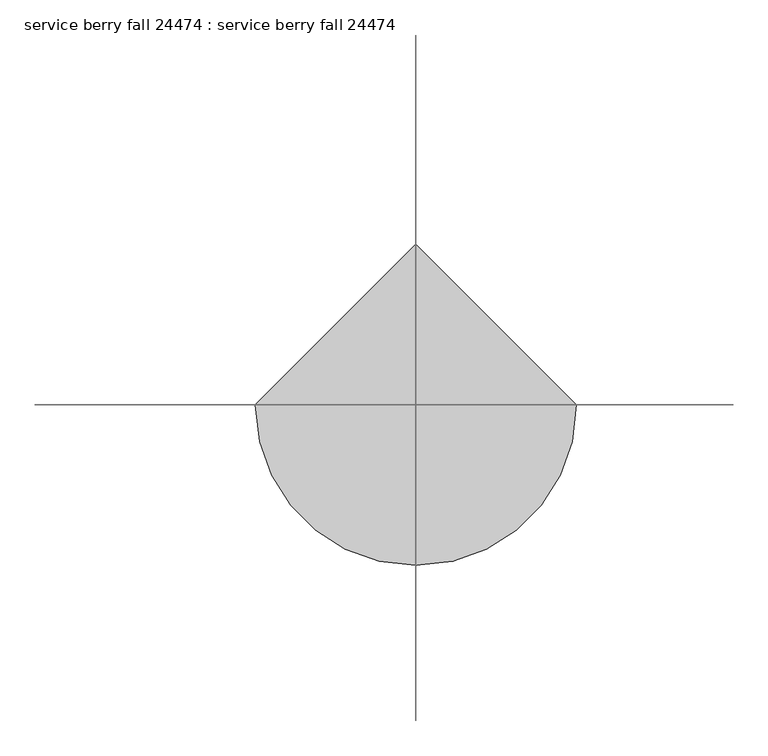
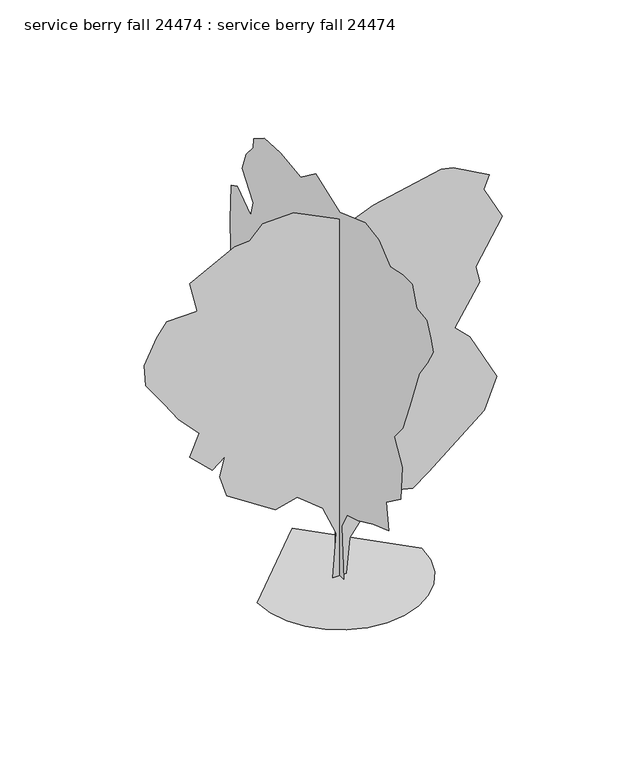
"""IFC4 building model written with IfcOpenShell, lengths in millimetres: proxy geometry, service berry fall 24474 : service berry fall 24474."""

import ifcopenshell
import ifcopenshell.guid

model = None  # the IFC model being written
_history = None  # IfcOwnerHistory: only IFC2X3 demands one
_inside = {}  # id of a spatial element -> (the spatial element, [elements in it])
_under = {}  # id of a project, library or spatial element -> (it, [spatial elements below it])
_declared = {}  # id of a project -> (the project, [libraries it declares])
_typed = {}  # id of a type object -> (the type object, [elements of that type])
_made_of = {}  # id of a material, layer set ... -> (it, [elements and type objects made of it])


def new_model(schema):
    """Start an empty IFC model of exactly this schema.

    Asked for "IFC4X3", IfcOpenShell would pick the latest addendum, in which some entities
    have other attributes; the version numbers below select the first issue.
    IFC2X3 requires an IfcOwnerHistory on every rooted entity: one is made here for all.
    """
    global model, _history
    if schema == "IFC4X3":
        model = ifcopenshell.file(schema_version=(4, 3, 0, 0))
    else:
        model = ifcopenshell.file(schema=schema)
    _inside.clear()
    _under.clear()
    _declared.clear()
    _typed.clear()
    _made_of.clear()
    _history = None
    if model.schema == "IFC2X3":
        org = make("IfcOrganization", Name="unknown")
        user = make(
            "IfcPersonAndOrganization",
            ThePerson=make("IfcPerson", FamilyName="unknown"),
            TheOrganization=org,
        )
        app = make(
            "IfcApplication",
            ApplicationDeveloper=org,
            Version="unknown",
            ApplicationFullName="unknown",
            ApplicationIdentifier="unknown",
        )
        _history = make(
            "IfcOwnerHistory",
            OwningUser=user,
            OwningApplication=app,
            ChangeAction="ADDED",
            CreationDate=0,
        )
    return model


def make(cls, **values):
    """One entity of the class cls with the attributes given. An attribute that is None is left unset."""
    return model.create_entity(
        cls, **{name: value for name, value in values.items() if value is not None}
    )


def rooted(cls, **values):
    """An entity with a GlobalId (a new one), such as an element, a storey or a relation."""
    return make(cls, GlobalId=ifcopenshell.guid.new(), OwnerHistory=_history, **values)


def si_unit(unit_type, name, prefix=None):
    """IfcSIUnit, for example si_unit("LENGTHUNIT", "METRE", prefix="MILLI")."""
    return make("IfcSIUnit", UnitType=unit_type, Prefix=prefix, Name=name)


def assignment(units):
    """IfcUnitAssignment: the units of a project."""
    return None if units is None else make("IfcUnitAssignment", Units=units)


def point(xyz):
    """IfcCartesianPoint."""
    return None if xyz is None else make("IfcCartesianPoint", Coordinates=xyz)


def direction(xyz):
    """IfcDirection."""
    return None if xyz is None else make("IfcDirection", DirectionRatios=xyz)


def frame(location, z_axis=None, x_axis=None):
    """IfcAxis2Placement3D, a coordinate frame: its origin and axes. An axis left out is left unset."""
    return make(
        "IfcAxis2Placement3D",
        Location=point(location),
        Axis=direction(z_axis),
        RefDirection=direction(x_axis),
    )


def origin():
    """The frame at (0, 0, 0) with its axes left unset."""
    return frame((0.0, 0.0, 0.0))


def place(relative_to, where):
    """IfcLocalPlacement: puts the frame where relative to a parent placement (None: the world)."""
    return make(
        "IfcLocalPlacement", PlacementRelTo=relative_to, RelativePlacement=where
    )


def context(
    kind, dimensions, precision=None, world=None, true_north=None, identifier=None
):
    """IfcGeometricRepresentationContext, for example the 3D "Model" context."""
    return make(
        "IfcGeometricRepresentationContext",
        ContextIdentifier=identifier,
        ContextType=kind,
        CoordinateSpaceDimension=dimensions,
        Precision=precision,
        WorldCoordinateSystem=world,
        TrueNorth=true_north,
    )


def project(units=None, contexts=None):
    """IfcProject with its units and contexts."""
    return rooted(
        "IfcProject",
        Name="project",
        RepresentationContexts=contexts,
        UnitsInContext=assignment(units),
    )


def spatial(cls, under=None, at=None, **own):
    """A site, building, storey or space (cls), placed at a placement, below another one or the project."""
    s = rooted(cls, ObjectPlacement=at, **own)
    if under is not None:
        _under.setdefault(under.id(), (under, []))[1].append(s)
    return s


def point_list(points):
    """IfcCartesianPointList2D or 3D."""
    cls = (
        "IfcCartesianPointList2D" if len(points[0]) == 2 else "IfcCartesianPointList3D"
    )
    return make(cls, CoordList=points)


def triangles(points, corners, closed=None, point_numbers=None):
    """IfcTriangulatedFaceSet: each triangle names its three corners, points numbered from 1."""
    return make(
        "IfcTriangulatedFaceSet",
        Coordinates=point_list(points),
        Closed=closed,
        CoordIndex=corners,
        PnIndex=point_numbers,
    )


def shape(context_of_items, identifier, shape_type, items):
    """IfcShapeRepresentation: the items that make up one representation, for example the "Body"."""
    return make(
        "IfcShapeRepresentation",
        ContextOfItems=context_of_items,
        RepresentationIdentifier=identifier,
        RepresentationType=shape_type,
        Items=items,
    )


def source(mapping_origin, context_of_items, identifier, shape_type, items):
    """IfcRepresentationMap: a shape defined once, which mapped items show again and again."""
    return make(
        "IfcRepresentationMap",
        MappingOrigin=mapping_origin,
        MappedRepresentation=shape(context_of_items, identifier, shape_type, items),
    )


def transform(
    local_origin,
    x_axis=None,
    y_axis=None,
    z_axis=None,
    scale=None,
    scale2=None,
    scale3=None,
    uniform=True,
):
    """IfcCartesianTransformationOperator3D, or its non-uniform kind. x_axis, y_axis, z_axis: its Axis1, 2, 3."""
    if uniform:
        return make(
            "IfcCartesianTransformationOperator3D",
            Axis1=direction(x_axis),
            Axis2=direction(y_axis),
            LocalOrigin=point(local_origin),
            Scale=scale,
            Axis3=direction(z_axis),
        )
    return make(
        "IfcCartesianTransformationOperator3DnonUniform",
        Axis1=direction(x_axis),
        Axis2=direction(y_axis),
        LocalOrigin=point(local_origin),
        Scale=scale,
        Axis3=direction(z_axis),
        Scale2=scale2,
        Scale3=scale3,
    )


def mapped(mapping_source, mapping_target):
    """IfcMappedItem: shows the shape of a source again, moved by a transform."""
    return make(
        "IfcMappedItem", MappingSource=mapping_source, MappingTarget=mapping_target
    )


def made_of(thing, what):
    """Note that an element or type object is made of a material, layer set ...; save() writes the relation."""
    if what is not None:
        _made_of.setdefault(what.id(), (what, []))[1].append(thing)
    return thing


def element(
    cls,
    number,
    at=None,
    inside=None,
    cuts=None,
    type_object=None,
    material=None,
    context=None,
    identifier="Body",
    shape_type=None,
    held_by="IfcProductDefinitionShape",
    body=None,
    shapes=None,
    **own,
):
    """One element of the class cls, such as IfcWall. Its Tag is "e" and its number.

    at: its placement. inside: the storey or other place that contains it. cuts: it is an
    opening in that element (IfcRelVoidsElement). A single representation is given by context,
    identifier, shape_type and body (its items); several are given by shapes. held_by: the class
    of the entity that holds the representations. save() writes the other relations.
    """
    e = rooted(cls, Tag="e%d" % number, ObjectPlacement=at, **own)
    if body is not None:
        shapes = [shape(context, identifier, shape_type, body)]
    if shapes is not None:
        e.Representation = make(held_by, Representations=shapes)
    if inside is not None:
        _inside.setdefault(inside.id(), (inside, []))[1].append(e)
    if cuts is not None:
        rooted(
            "IfcRelVoidsElement", RelatingBuildingElement=cuts, RelatedOpeningElement=e
        )
    if type_object is not None:
        _typed.setdefault(type_object.id(), (type_object, []))[1].append(e)
    return made_of(e, material)


def aggregate(whole, parts):
    """IfcRelAggregates: a whole, such as a stair, and the parts it consists of."""
    return rooted("IfcRelAggregates", RelatingObject=whole, RelatedObjects=parts)


def save(model, path):
    """Write the relations noted so far, then the file.

    IfcRelAggregates (storeys below a building ...), IfcRelContainedInSpatialStructure (elements
    in a storey), IfcRelDefinesByType, IfcRelAssociatesMaterial and IfcRelDeclares: one each for
    every whole, place, type object, material and project.
    """
    for whole, parts in _under.values():
        aggregate(whole, parts)
    for where, things in _inside.values():
        rooted(
            "IfcRelContainedInSpatialStructure",
            RelatedElements=things,
            RelatingStructure=where,
        )
    for kind, things in _typed.values():
        rooted("IfcRelDefinesByType", RelatedObjects=things, RelatingType=kind)
    for what, things in _made_of.values():
        rooted("IfcRelAssociatesMaterial", RelatedObjects=things, RelatingMaterial=what)
    for by, libraries in _declared.values():
        rooted("IfcRelDeclares", RelatingContext=by, RelatedDefinitions=libraries)
    model.write(path)


def service_berry_fall_24474_service_berry_fall_24474_c2e3b044(model_context):
    return source(origin(), model_context, "Body", "Tessellation", [
        triangles([(-1569.2053802, 0.0, 0.0921994), (-1527.7195404, -359.5569775, 0.0921994), (-1409.5715195, -689.7541191, 0.0921994), (-1224.2203331, -981.1298658, 0.0921994), (-981.1298658, -1224.2203331, 0.0921994), (-689.7541191, -1409.5715195, 0.0921994), (-359.5569775, -1527.7195404, 0.0921994), (6.86e-05, -1569.2053802, 0.0921994), (359.5569775, -1527.7195404, 0.0921994), (689.7541191, -1409.5715195, 0.0921994), (981.1298658, -1224.2203331, 0.0921994), (1224.2229492, -981.1298658, 0.0921994), (1409.5715195, -689.7541191, 0.0921994), (1527.7195404, -359.5569775, 0.0921994), (1569.2053802, 0.0001372, 0.0921994), (-0.0002058, 1569.2053802, 0.0921994), (-1.69e-05, -141.5174793, 0.1472589), (0.0001147, -69.7424863, 1032.2016031), (0.000133, -256.3848048, 1371.9187305), (0.0001024, -615.3550266, 1474.4812202), (7.03e-05, -1115.345874, 1705.2476578), (3.21e-05, -1615.3367214, 1884.7314697), (0.0001039, -1538.4155445, 2410.3636299), (8.87e-05, -2012.7650791, 2756.5067459), (0.0001635, -2064.0477047, 3435.9815506), (0.000217, -1897.3831684, 3718.0227654), (0.0002491, -1794.8206787, 3884.6974754), (0.0002552, -2089.6888721, 4230.8484398), (0.000298, -2307.6334179, 4807.7579933), (0.0003614, -2623.385511, 5655.5326996), (0.0003744, -2884.5480583, 6025.68685), (0.0003913, -3089.67827, 6371.8378143), (0.0004295, -2999.9401428, 6602.5964035), (0.0004784, -2871.721225, 6884.6379089), (0.0005227, -2551.224218, 6935.9202438), (0.0005869, -2397.3740158, 7320.5264191), (0.0006248, -2079.5720478, 7320.8822113), (0.0006638, -1662.9541637, 7231.2458221), (0.0007467, -1282.8054199, 7546.7643539), (0.0008078, -843.8836647, 7619.9924423), (0.0008724, -0.5889314, 7319.3073074), (0.0010019, 789.2051708, 7615.6235229), (0.0010175, 1284.1033058, 7251.4131958), (0.001108, 1961.5257648, 7333.3535431), (0.0011676, 2487.1577797, 7307.7248749), (0.0011829, 2846.1178459, 7076.9407059), (0.0011624, 2859.3260513, 6891.47005), (0.0011569, 3089.7038498, 6615.4235275), (0.0011294, 3217.9227676, 6256.4454391), (0.0010299, 2847.8197769, 5791.7784531), (0.0010042, 2946.0922668, 5477.7836655), (0.0010936, 3377.5871498, 5796.1217926), (0.0011065, 3589.7021095, 5692.3630096), (0.0010255, 3615.3560669, 4987.2339569), (0.0008843, 3582.2092529, 3836.2597343), (0.0007687, 3089.7038498, 3359.0705475), (0.0006236, 2628.1860901, 2602.6591599), (0.0005208, 2040.694915, 2327.8239006), (0.0004249, 1431.5069538, 2133.0466908), (0.0004088, 1159.6180264, 2269.3404064), (0.0003546, 948.7221056, 2025.7546932), (0.0003347, 1038.465247, 1769.3469429), (0.0003041, 974.3633457, 1577.0438553), (0.0002185, 601.9539914, 1230.895507), (0.0002096, 314.8453897, 1443.1579868), (0.0001473, 143.6297414, 1092.3639919), (1.53e-05, 128.0166319, 0.0873663), (-131.1532773, 5.7e-06, 1.11e-05), (-67.2957107, -0.0001014, 875.4050692), (-322.2342556, -0.0001611, 1469.2590099), (-813.1217342, -0.0001862, 1859.996933), (-1229.3790298, -0.000155, 1751.1580822), (-2156.2470188, -0.0001869, 2358.9337749), (-2290.3894123, -0.0002327, 2792.1938118), (-2194.7076073, -0.0002815, 3166.6148529), (-2430.1146046, -0.0002486, 2976.2674599), (-2861.3579041, -0.0002784, 3384.5466087), (-2681.1450668, -0.0003364, 3804.8398499), (-3066.4881157, -0.0003688, 4217.8689995), (-3348.5293304, -0.0004053, 4628.1294228), (-3694.6802948, -0.0004483, 5115.3011398), (-3724.9569351, -0.0004968, 5533.4604996), (-3491.4551994, -0.000565, 6019.7430267), (-3297.2469955, -0.0006032, 6269.1202469), (-2715.1302017, -0.0006298, 6278.9242996), (-2861.3579041, -0.0006956, 6884.5105911), (-2002.4019035, -0.0007866, 7333.2012268), (-1714.1578697, -0.0008013, 7350.6001648), (-1463.9504677, -0.0008423, 7602.441188), (-879.4385439, -0.0008697, 7618.3158005), (233.9073432, -0.0008534, 7073.1560532), (638.5782457, -0.0008914, 7243.4630997), (1933.428352, -0.0009801, 7512.7030609), (2164.1946442, -0.0009841, 7461.4201447), (2852.671225, -0.0009686, 7079.2521927), (2750.5632133, -0.0009338, 6825.0491043), (3100.854332, -0.0008692, 6154.4644547), (2597.0202599, -0.000747, 5314.284343), (2668.3182335, -0.0007111, 4986.9549042), (2193.0693352, -0.0006001, 4229.7307755), (2484.1352898, -0.0005783, 3940.602784), (2995.342749, -0.0004845, 2966.2343513), (2760.2152405, -0.0004028, 2366.9321239), (1689.8424934, -0.0002511, 1487.1532665), (1388.3447628, -0.0002125, 1273.8112015), (830.8839495, -0.0002044, 1410.2319443), (535.8861128, -0.0001613, 1156.8088228), (193.8940152, -9.15e-05, 696.3936121), (121.4733449, -5.3e-06, 0.0)], [[15, 16, 1], [14, 15, 1], [14, 1, 2], [13, 14, 2], [13, 2, 3], [13, 3, 4], [12, 13, 4], [11, 12, 4], [11, 4, 5], [11, 5, 6], [11, 6, 7], [11, 7, 8], [11, 8, 9], [11, 9, 10], [67, 17, 18], [66, 67, 18], [63, 64, 65], [21, 22, 23], [66, 18, 19], [65, 66, 19], [35, 36, 37], [51, 52, 53], [51, 53, 54], [62, 63, 65], [61, 62, 65], [48, 49, 50], [41, 42, 43], [33, 34, 35], [47, 48, 50], [51, 54, 55], [51, 55, 56], [45, 46, 47], [31, 32, 33], [31, 33, 35], [30, 31, 35], [35, 37, 38], [30, 35, 38], [29, 30, 38], [23, 24, 25], [23, 25, 26], [23, 26, 27], [44, 45, 47], [44, 47, 50], [43, 44, 50], [58, 59, 60], [41, 43, 50], [41, 50, 51], [41, 51, 56], [41, 56, 57], [41, 57, 58], [41, 58, 60], [40, 41, 60], [39, 40, 60], [38, 39, 60], [29, 38, 60], [28, 29, 60], [27, 28, 60], [23, 27, 60], [23, 60, 61], [21, 23, 61], [20, 21, 61], [20, 61, 65], [20, 65, 19], [109, 68, 69], [108, 109, 69], [107, 108, 69], [107, 69, 70], [94, 95, 96], [75, 76, 77], [75, 77, 78], [85, 86, 87], [106, 107, 70], [96, 97, 98], [85, 87, 88], [83, 84, 85], [101, 102, 103], [101, 103, 104], [100, 101, 104], [104, 105, 106], [100, 104, 106], [100, 106, 70], [100, 70, 71], [94, 96, 98], [93, 94, 98], [92, 93, 98], [91, 92, 98], [71, 72, 73], [100, 71, 73], [100, 73, 74], [100, 74, 75], [100, 75, 78], [99, 100, 78], [98, 99, 78], [91, 98, 78], [90, 91, 78], [89, 90, 78], [88, 89, 78], [85, 88, 78], [85, 78, 79], [85, 79, 80], [83, 85, 80], [83, 80, 81], [82, 83, 81]], closed=False),
    ])


if __name__ == "__main__":
    model = new_model("IFC4")
    model_context = context("Model", 3, world=origin())
    ifc_project = project(units=[si_unit("LENGTHUNIT", "METRE", prefix="MILLI")], contexts=[model_context])
    site = spatial("IfcSite", under=ifc_project)
    building = spatial("IfcBuilding", under=site)
    placement = place(None, origin())
    service_berry_fall_24474_service_berry_fall_24474_shape = service_berry_fall_24474_service_berry_fall_24474_c2e3b044(model_context)
    element("IfcBuildingElementProxy", 1, Name="service berry fall 24474 : service berry fall 24474", ObjectType="service berry fall 24474 : service berry fall 24474", at=placement, inside=building, context=model_context, shape_type="MappedRepresentation", body=[
        mapped(service_berry_fall_24474_service_berry_fall_24474_shape, transform((0.0, 0.0, 0.0), x_axis=(1.0, 0.0, 0.0), y_axis=(0.0, 1.0, 0.0), z_axis=(0.0, 0.0, 1.0))),
    ])
    save(model, "model.ifc")

# Revit data of these elements
# Type "service berry fall 24474 : service berry fall 24474"
#   built-in parameter 1005195 = "RPC-16-FVGU-8VG0-7PL0-4000-ST1L-LVER-AU"
#   Height = 0
